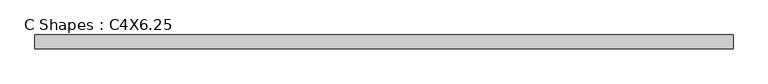
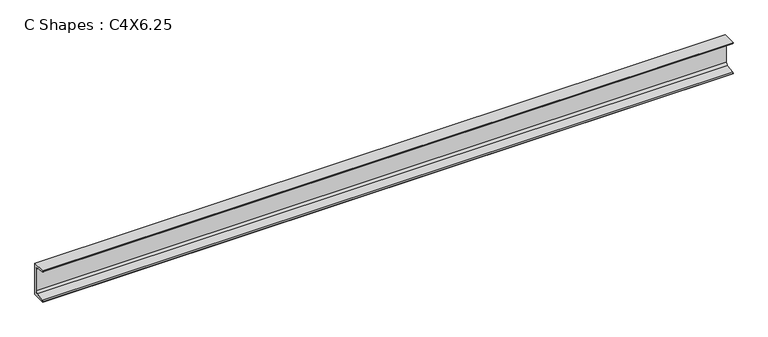
"""IFC4 building model written with IfcOpenShell, lengths in millimetres: beam geometry, C Shapes : C4X6.25."""

from ifc_helpers import new_model, si_unit, point, frame, frame_2d, origin, place, context, project, spatial, polyline, circle_curve, trimmed, segment, composite_curve, outline, extrude, source, transform, mapped, element, save


def c_shapes_c4x6_25_cfd2a1e4(model_context):
    return source(origin(), model_context, "Body", "SweptSolid", [
        extrude(outline(composite_curve([segment(polyline([(11.049, 50.8), (11.049, -50.8), (-30.861, -50.8), (-30.861, -49.7865772)]), True, "CONTINUOUS"), segment(trimmed(circle_curve(frame_2d((-27.4066, -49.7865772)), 3.4544), [point((-30.861, -49.7865772))], [point((-27.9743618, -46.379155))], False, "CARTESIAN"), True, "CONTINUOUS"), segment(polyline([(-27.9743618, -46.379155), (-0.9980765, -41.8842311)]), True, "CONTINUOUS"), segment(trimmed(circle_curve(frame_2d((-2.1336, -35.0693868)), 6.9088), [point((-0.9980765, -41.8842311))], [point((4.7752, -35.0693868))], True, "CARTESIAN"), True, "CONTINUOUS"), segment(polyline([(4.7752, -35.0693868), (4.7752, 35.0693868)]), True, "CONTINUOUS"), segment(trimmed(circle_curve(frame_2d((-2.1336, 35.0693868)), 6.9088), [point((4.7752, 35.0693868))], [point((-0.9980765, 41.8842311))], True, "CARTESIAN"), True, "CONTINUOUS"), segment(polyline([(-0.9980765, 41.8842311), (-27.9743618, 46.379155)]), True, "CONTINUOUS"), segment(trimmed(circle_curve(frame_2d((-27.4066, 49.7865772)), 3.4544), [point((-27.9743618, 46.379155))], [point((-30.861, 49.7865772))], False, "CARTESIAN"), True, "CONTINUOUS"), segment(polyline([(-30.861, 49.7865772), (-30.861, 50.8), (11.049, 50.8)]), True, "CONTINUOUS")], self_intersect=False)), frame((-1063.2174237, 0.0, 0.0), z_axis=(1.0, 0.0, 0.0), x_axis=(0.0, 1.0, 0.0)), (0.0, 0.0, 1.0), 2126.4348474),
    ])


if __name__ == "__main__":
    model = new_model("IFC4")
    model_context = context("Model", 3, world=origin())
    ifc_project = project(units=[si_unit("LENGTHUNIT", "METRE", prefix="MILLI")], contexts=[model_context])
    site = spatial("IfcSite", under=ifc_project)
    building = spatial("IfcBuilding", under=site)
    placement = place(None, origin())
    c_shapes_c4x6_25_shape = c_shapes_c4x6_25_cfd2a1e4(model_context)
    element("IfcBeam", 1, ObjectType="C Shapes : C4X6.25", at=placement, inside=building, context=model_context, shape_type="MappedRepresentation", body=[
        mapped(c_shapes_c4x6_25_shape, transform((0.0, 0.0, 0.0), x_axis=(1.0, 0.0, 0.0), y_axis=(0.0, 1.0, 0.0), z_axis=(0.0, 0.0, 1.0))),
    ])
    save(model, "model.ifc")

# Revit data of these elements
# Type "C Shapes : C4X6.25"
#   Section Name Key = "ChannelsC4X6.25"
#   Assembly Code = "B10"
#   Width = 1.650"
#   Web Thickness = 0.247"
#   Web Fillet = 0.272"
#   Warping Constant = 1.03 in⁶
#   Torsional Moment of Inertia = 0.0487 in⁴
#   Sloped Flange Angle = 9.46°
#   Section Area = 1.77 in²
#   Plastic Modulus weak axis = 0.569 in³
#   Plastic Modulus strong axis = 2.43 in³
#   Nominal Weight = 6.25 lbf/ft
#   Moment of Inertia weak axis = 0.345 in⁴
#   Moment of Inertia strong axis = 4.00 in⁴
#   Height = 4.000"
#   Flange Thickness Location = 0.7015"
#   Flange Thickness = 0.272"
#   Flange Fillet = 0.136"
#   Elastic Modulus weak axis = 0.284 in³
#   Elastic Modulus strong axis = 2.00 in³
#   Centroid Vertical = 2.000"
#   Centroid Horizontal = 0.435"
#   Length [instance default] = 5' - 0"
#   Structural Material [instance default] = Steel ASTM A36
#   Principal Axes Angle = 0
#   Bolt Spacing = 0
# Element 1 (IfcBeam, "C Shapes : C4X6.25")
#   Materials on its faces: "Steel ASTM A36"
# Materials
#   "Steel ASTM A36": class "Metal", colour RGB 199 199 199, transparency 0, Description = "Structural steel, ASTM A36 Grade B, mill finish", Cost = 0
